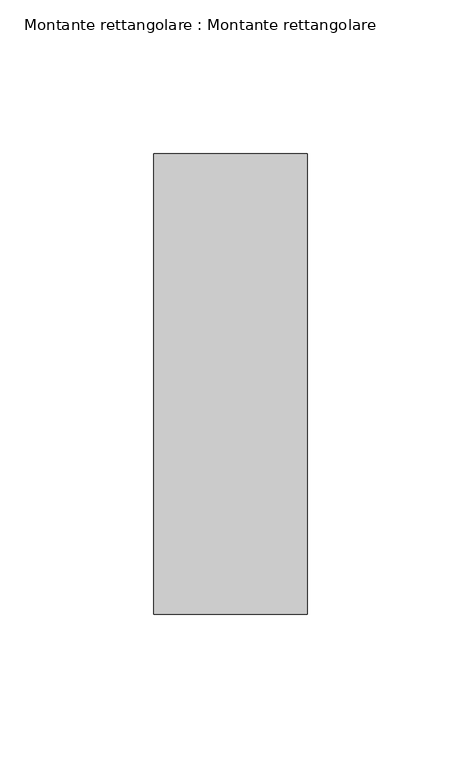
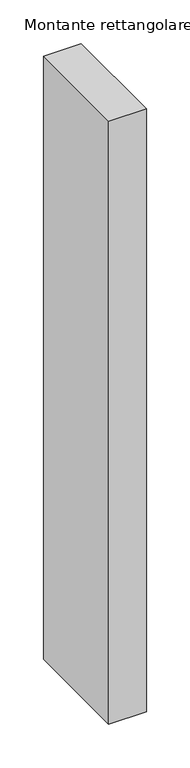
"""IFC4 building model written with IfcOpenShell, lengths in millimetres: member geometry, Montante rettangolare : Montante rettangolare."""

from ifc_helpers import new_model, si_unit, frame, origin, place, context, project, spatial, polyline, outline, extrude, source, transform, mapped, element, save


def montante_rettangolare_montante_rettangolare_a28e36f6(model_context):
    return source(origin(), model_context, "Body", "SweptSolid", [
        extrude(outline(polyline([(25.0, 75.0), (25.0, -75.0), (-25.0, -75.0), (-25.0, 75.0), (25.0, 75.0)])), frame((0.0, 0.0, -845.0), z_axis=(0.0, 0.0, 1.0), x_axis=(1.0, 0.0, 0.0)), (0.0, 0.0, 1.0), 845.0),
    ])


if __name__ == "__main__":
    model = new_model("IFC4")
    model_context = context("Model", 3, world=origin())
    ifc_project = project(units=[si_unit("LENGTHUNIT", "METRE", prefix="MILLI")], contexts=[model_context])
    site = spatial("IfcSite", under=ifc_project)
    building = spatial("IfcBuilding", under=site)
    placement = place(None, origin())
    montante_rettangolare_montante_rettangolare_shape = montante_rettangolare_montante_rettangolare_a28e36f6(model_context)
    element("IfcMember", 1, ObjectType="Montante rettangolare : Montante rettangolare", at=placement, inside=building, context=model_context, shape_type="MappedRepresentation", body=[
        mapped(montante_rettangolare_montante_rettangolare_shape, transform((0.0, 0.0, 0.0), x_axis=(1.0, 0.0, 0.0), y_axis=(0.0, 1.0, 0.0), z_axis=(0.0, 0.0, 1.0))),
    ])
    save(model, "model.ifc")

# Revit data of these elements
# Type "Montante rettangolare : Montante rettangolare"
#   built-in parameter 1007304 = 0.492126 (stored number, unit not read)
#   built-in parameter 1007301 = 0.082021 (stored number, unit not read)
#   built-in parameter 1007300 = 0.082021 (stored number, unit not read)
# Element 1 (IfcMember, "Montante rettangolare : Montante rettangolare")
#   Materials on its faces: "Acciaio"
# Materials
#   "Acciaio": class "Metallo", colour RGB 247 247 247, transparency 0, Description = "Acciaio, finitura zigrinata", Cost = 0
